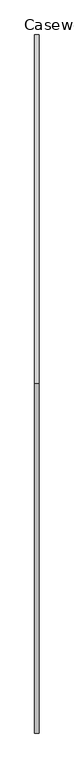
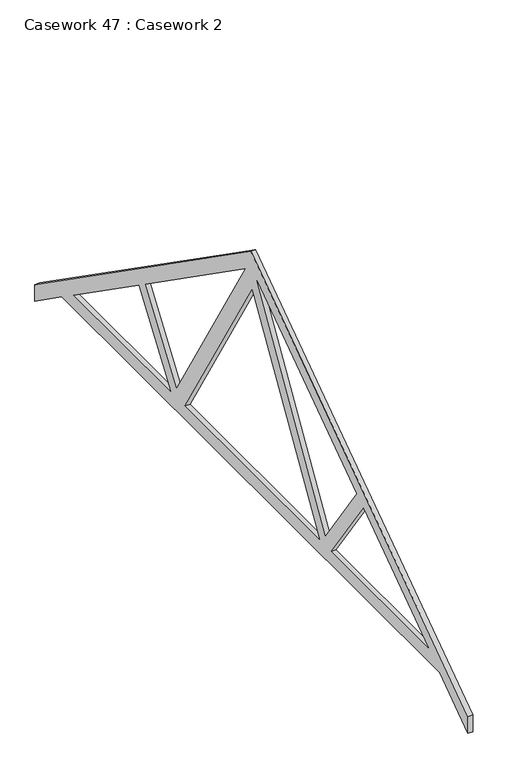
"""IFC4 building model written with IfcOpenShell, lengths in millimetres: furniture geometry, Casework 47 : Casework 2."""

from ifc_helpers import new_model, si_unit, frame, origin, place, context, project, spatial, polyline, outline, extrude, source, transform, mapped, element, save


def casework_47_casework_2_612639c6(model_context):
    return source(origin(), model_context, "Body", "SweptSolid", [
        extrude(outline(polyline([(6583.1149316, 5265.0), (-277.3850684, 5265.0), (-786.6126654, 4908.4349979), (-786.6126654, 5091.5511862), (3152.8649316, 7850.0030963), (7073.1149316, 5105.0144946), (7073.1149316, 4921.8983063), (6583.1149316, 5265.0)]), holes=[polyline([(4612.3149663, 5415.0), (6368.8927306, 5415.0), (5190.2113591, 6240.3215815), (4612.3149663, 5415.0)]), polyline([(4346.6651995, 5415.0), (3129.0956471, 7441.3760243), (1911.5260948, 5415.0), (4346.6651995, 5415.0)]), polyline([(4504.5438357, 5522.6038939), (5067.3385525, 6326.3580469), (3262.0771677, 7590.415677), (4504.5438357, 5522.6038939)]), polyline([(1693.4148969, 5415.0), (1115.5185041, 6240.3215815), (-63.1628674, 5415.0), (1693.4148969, 5415.0)]), polyline([(1801.1860276, 5522.6038939), (3043.6526956, 7590.415677), (1238.3913108, 6326.3580469), (1801.1860276, 5522.6038939)])]), frame((-10901.5247381, 0.0, 0.0), z_axis=(1.0, 0.0, 0.0), x_axis=(0.0, 1.0, 0.0)), (0.0, 0.0, 1.0), 49.6351915),
    ])


if __name__ == "__main__":
    model = new_model("IFC4")
    model_context = context("Model", 3, world=origin())
    ifc_project = project(units=[si_unit("LENGTHUNIT", "METRE", prefix="MILLI")], contexts=[model_context])
    site = spatial("IfcSite", under=ifc_project)
    building = spatial("IfcBuilding", under=site)
    placement = place(None, origin())
    casework_47_casework_2_shape = casework_47_casework_2_612639c6(model_context)
    element("IfcFurniture", 1, ObjectType="Casework 47 : Casework 2", at=placement, inside=building, context=model_context, shape_type="MappedRepresentation", body=[
        mapped(casework_47_casework_2_shape, transform((0.0, 0.0, 0.0), x_axis=(1.0, 0.0, 0.0), y_axis=(0.0, 1.0, 0.0), z_axis=(0.0, 0.0, 1.0))),
    ])
    save(model, "model.ifc")

# Revit data of these elements
# Element 1 (IfcFurniture, "Casework 47 : Casework 2")
#   Materials on its faces: "Softwood, Lumber"
# Materials
#   "Softwood, Lumber": class "Wood", colour RGB 205 156 65, transparency 0, Description = "Pinus Echinata", Cost = 0
